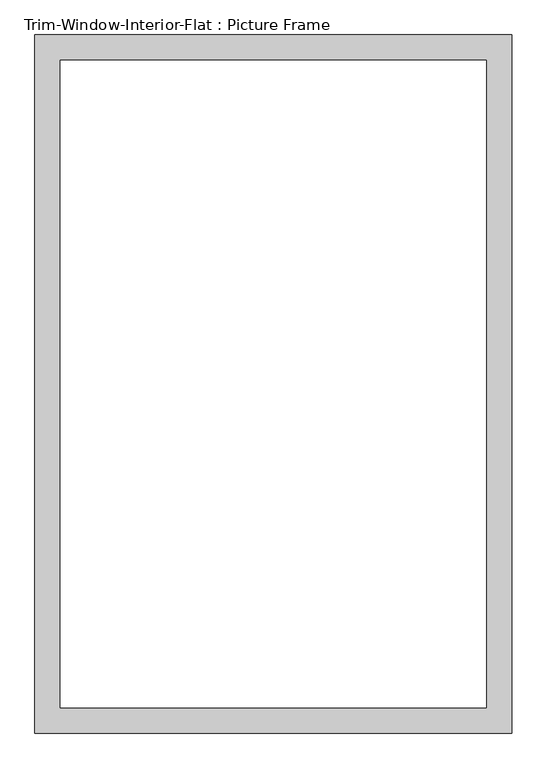
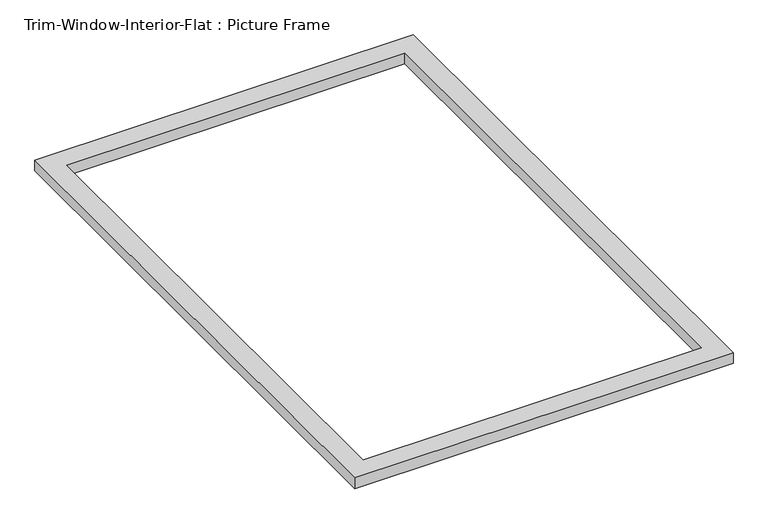
"""IFC4 building model written with IfcOpenShell, lengths in millimetres: proxy geometry, Trim-Window-Interior-Flat : Picture Frame."""

from ifc_helpers import new_model, si_unit, origin, origin_with_axes, place, context, project, spatial, polyline, outline, extrude, source, transform, mapped, element, save


def trim_window_interior_flat_picture_frame_3ffcdbcf(model_context):
    return source(origin(), model_context, "Body", "SweptSolid", [
        extrude(outline(polyline([(533.4, 44.45), (533.4, -1517.65), (-533.4, -1517.65), (-533.4, 44.45), (533.4, 44.45)]), holes=[polyline([(476.25, -12.7), (-476.25, -12.7), (-476.25, -1460.5), (476.25, -1460.5), (476.25, -12.7)])]), origin_with_axes(), (0.0, 0.0, 1.0), 31.75),
    ])


if __name__ == "__main__":
    model = new_model("IFC4")
    model_context = context("Model", 3, world=origin())
    ifc_project = project(units=[si_unit("LENGTHUNIT", "METRE", prefix="MILLI")], contexts=[model_context])
    site = spatial("IfcSite", under=ifc_project)
    building = spatial("IfcBuilding", under=site)
    placement = place(None, origin())
    trim_window_interior_flat_picture_frame_shape = trim_window_interior_flat_picture_frame_3ffcdbcf(model_context)
    element("IfcBuildingElementProxy", 1, Name="Trim-Window-Interior-Flat : Picture Frame", ObjectType="Trim-Window-Interior-Flat : Picture Frame", at=placement, inside=building, context=model_context, shape_type="MappedRepresentation", body=[
        mapped(trim_window_interior_flat_picture_frame_shape, transform((0.0, 0.0, 0.0), x_axis=(1.0, 0.0, 0.0), y_axis=(0.0, 1.0, 0.0), z_axis=(0.0, 0.0, 1.0))),
    ])
    save(model, "model.ifc")

# Revit data of these elements
# Type "Trim-Window-Interior-Flat : Picture Frame"
#   Trim Thickness_Picture Frame = 0' - 1 1/4"
#   Trim Width = 0' - 2 1/4"
#   Trim Thickness_with Sill = 0' - 0 3/4"
#   Sill Thickness = 0' - 1 1/4"
#   Opening Width [instance default] = 2' - 0"
#   Opening Height [instance default] = 3' - 0"
#   Default Elevation = 4' - 0"
#   Sill = no
#   Picture Frame = yes
#   Trim Material [instance default] = none
# Element 1 (IfcBuildingElementProxy, "Trim-Window-Interior-Flat : Picture Frame")
#   Opening Width = 3' - 2 1/2"
#   Opening Height = 4' - 10"
#   Trim Material = 1X WOOD COMPOSITE TRIM
#   Materials on its faces: "1X WOOD COMPOSITE TRIM"
# Materials
#   "1X WOOD COMPOSITE TRIM": class "Generic", colour RGB 88 61 61, transparency 0, Cost = 0
